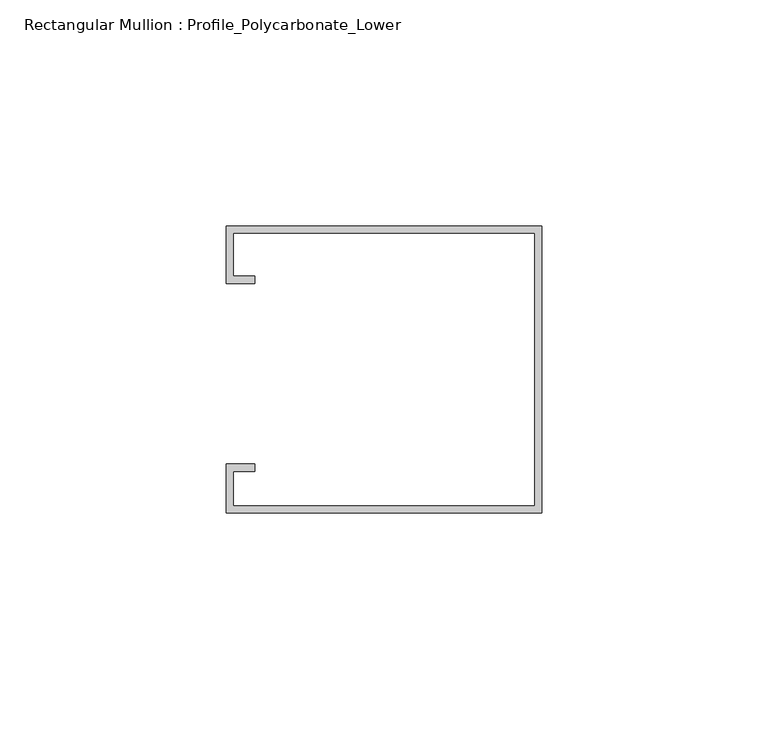
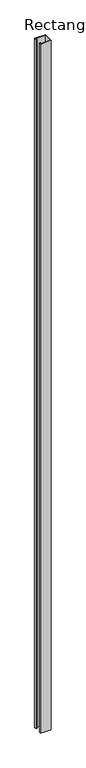
"""IFC4 building model written with IfcOpenShell, lengths in millimetres: member geometry, Rectangular Mullion : Profile_Polycarbonate_Lower."""

from ifc_helpers import new_model, si_unit, frame, origin, place, context, project, spatial, polyline, outline, extrude, source, transform, mapped, element, save


def rectangular_mullion_profile_polycarbonate_lower_528e47e7(model_context):
    return source(origin(), model_context, "Body", "SweptSolid", [
        extrude(outline(polyline([(0.0, 32.7), (0.0, -30.8), (-69.85, -30.8), (-69.85, -20.0), (-63.5, -20.0), (-63.5, -21.5875), (-68.2625, -21.5875), (-68.2625, -29.2125), (-1.5875, -29.2125), (-1.5875, 31.1125), (-68.2625, 31.1125), (-68.2625, 21.5875), (-63.5, 21.5875), (-63.5, 20.0), (-69.85, 20.0), (-69.85, 32.7), (0.0, 32.7)])), frame((0.0, 0.0, -4756.15), z_axis=(0.0, 0.0, 1.0), x_axis=(1.0, 0.0, 0.0)), (0.0, 0.0, 1.0), 4756.15),
    ])


if __name__ == "__main__":
    model = new_model("IFC4")
    model_context = context("Model", 3, world=origin())
    ifc_project = project(units=[si_unit("LENGTHUNIT", "METRE", prefix="MILLI")], contexts=[model_context])
    site = spatial("IfcSite", under=ifc_project)
    building = spatial("IfcBuilding", under=site)
    placement = place(None, origin())
    rectangular_mullion_profile_polycarbonate_lower_shape = rectangular_mullion_profile_polycarbonate_lower_528e47e7(model_context)
    element("IfcMember", 1, ObjectType="Rectangular Mullion : Profile_Polycarbonate_Lower", at=placement, inside=building, context=model_context, shape_type="MappedRepresentation", body=[
        mapped(rectangular_mullion_profile_polycarbonate_lower_shape, transform((0.0, 0.0, 0.0), x_axis=(1.0, 0.0, 0.0), y_axis=(0.0, 1.0, 0.0), z_axis=(0.0, 0.0, 1.0))),
    ])
    save(model, "model.ifc")

# Revit data of these elements
# Type "Rectangular Mullion : Profile_Polycarbonate_Lower"
#   built-in parameter 1007322 = 0.208333 (stored number, unit not read)
#   built-in parameter 1007321 = 0 (stored number, unit not read)
#   built-in parameter 1007320 = 0.00520833 (stored number, unit not read)
